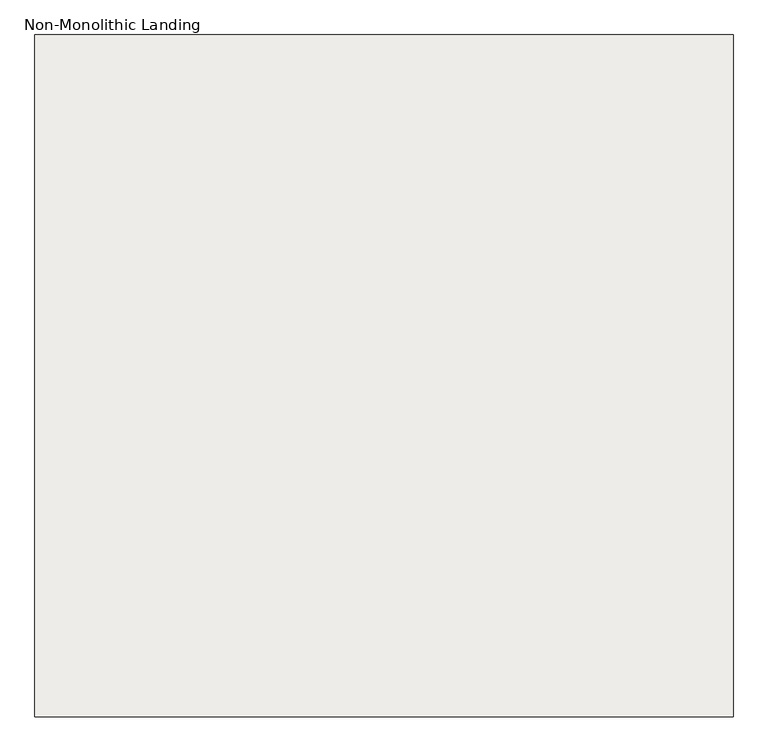
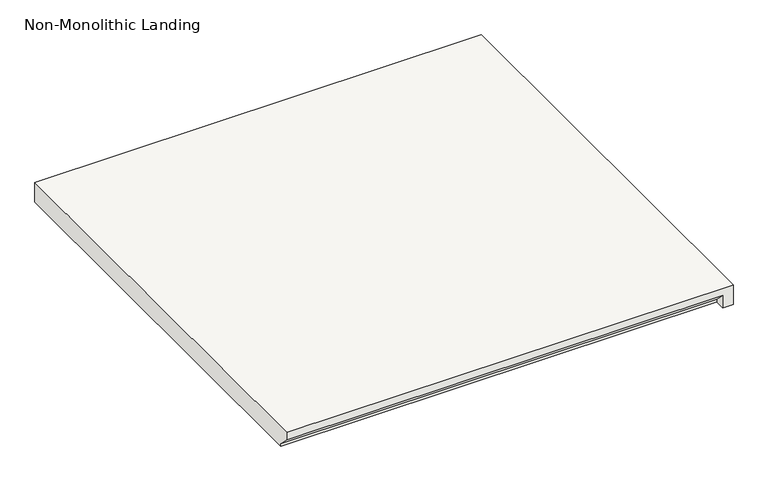
"""IFC4 building model written with IfcOpenShell, lengths in millimetres: slab geometry, Non-Monolithic Landing."""

import ifcopenshell
import ifcopenshell.guid

model = None  # the IFC model being written
_history = None  # IfcOwnerHistory: only IFC2X3 demands one
_inside = {}  # id of a spatial element -> (the spatial element, [elements in it])
_under = {}  # id of a project, library or spatial element -> (it, [spatial elements below it])
_declared = {}  # id of a project -> (the project, [libraries it declares])
_typed = {}  # id of a type object -> (the type object, [elements of that type])
_made_of = {}  # id of a material, layer set ... -> (it, [elements and type objects made of it])


def new_model(schema):
    """Start an empty IFC model of exactly this schema.

    Asked for "IFC4X3", IfcOpenShell would pick the latest addendum, in which some entities
    have other attributes; the version numbers below select the first issue.
    IFC2X3 requires an IfcOwnerHistory on every rooted entity: one is made here for all.
    """
    global model, _history
    if schema == "IFC4X3":
        model = ifcopenshell.file(schema_version=(4, 3, 0, 0))
    else:
        model = ifcopenshell.file(schema=schema)
    _inside.clear()
    _under.clear()
    _declared.clear()
    _typed.clear()
    _made_of.clear()
    _history = None
    if model.schema == "IFC2X3":
        org = make("IfcOrganization", Name="unknown")
        user = make(
            "IfcPersonAndOrganization",
            ThePerson=make("IfcPerson", FamilyName="unknown"),
            TheOrganization=org,
        )
        app = make(
            "IfcApplication",
            ApplicationDeveloper=org,
            Version="unknown",
            ApplicationFullName="unknown",
            ApplicationIdentifier="unknown",
        )
        _history = make(
            "IfcOwnerHistory",
            OwningUser=user,
            OwningApplication=app,
            ChangeAction="ADDED",
            CreationDate=0,
        )
    return model


def make(cls, **values):
    """One entity of the class cls with the attributes given. An attribute that is None is left unset."""
    return model.create_entity(
        cls, **{name: value for name, value in values.items() if value is not None}
    )


def rooted(cls, **values):
    """An entity with a GlobalId (a new one), such as an element, a storey or a relation."""
    return make(cls, GlobalId=ifcopenshell.guid.new(), OwnerHistory=_history, **values)


def si_unit(unit_type, name, prefix=None):
    """IfcSIUnit, for example si_unit("LENGTHUNIT", "METRE", prefix="MILLI")."""
    return make("IfcSIUnit", UnitType=unit_type, Prefix=prefix, Name=name)


def assignment(units):
    """IfcUnitAssignment: the units of a project."""
    return None if units is None else make("IfcUnitAssignment", Units=units)


def point(xyz):
    """IfcCartesianPoint."""
    return None if xyz is None else make("IfcCartesianPoint", Coordinates=xyz)


def direction(xyz):
    """IfcDirection."""
    return None if xyz is None else make("IfcDirection", DirectionRatios=xyz)


def frame(location, z_axis=None, x_axis=None):
    """IfcAxis2Placement3D, a coordinate frame: its origin and axes. An axis left out is left unset."""
    return make(
        "IfcAxis2Placement3D",
        Location=point(location),
        Axis=direction(z_axis),
        RefDirection=direction(x_axis),
    )


def origin():
    """The frame at (0, 0, 0) with its axes left unset."""
    return frame((0.0, 0.0, 0.0))


def place(relative_to, where):
    """IfcLocalPlacement: puts the frame where relative to a parent placement (None: the world)."""
    return make(
        "IfcLocalPlacement", PlacementRelTo=relative_to, RelativePlacement=where
    )


def context(
    kind, dimensions, precision=None, world=None, true_north=None, identifier=None
):
    """IfcGeometricRepresentationContext, for example the 3D "Model" context."""
    return make(
        "IfcGeometricRepresentationContext",
        ContextIdentifier=identifier,
        ContextType=kind,
        CoordinateSpaceDimension=dimensions,
        Precision=precision,
        WorldCoordinateSystem=world,
        TrueNorth=true_north,
    )


def project(units=None, contexts=None):
    """IfcProject with its units and contexts."""
    return rooted(
        "IfcProject",
        Name="project",
        RepresentationContexts=contexts,
        UnitsInContext=assignment(units),
    )


def spatial(cls, under=None, at=None, **own):
    """A site, building, storey or space (cls), placed at a placement, below another one or the project."""
    s = rooted(cls, ObjectPlacement=at, **own)
    if under is not None:
        _under.setdefault(under.id(), (under, []))[1].append(s)
    return s


def faces_of(points, faces, orient=None, outer=None):
    """IfcFace entities. A face is a list of loops; a loop is a list of indices into points, from 0.

    orient and outer hold one flag for each loop. By default every Orientation is true, the
    first loop of a face is its IfcFaceOuterBound and the others are IfcFaceBound.
    """
    made = []
    for i, loops in enumerate(faces):
        bounds = []
        for j, loop in enumerate(loops):
            is_outer = j == 0 if outer is None else outer[i][j]
            bounds.append(
                make(
                    "IfcFaceOuterBound" if is_outer else "IfcFaceBound",
                    Bound=make("IfcPolyLoop", Polygon=[points[k] for k in loop]),
                    Orientation=True if orient is None else orient[i][j],
                )
            )
        made.append(make("IfcFace", Bounds=bounds))
    return made


def faceted_brep(points, faces, orient=None, outer=None, voids=None):
    """IfcFacetedBrep: a solid bounded by flat faces; with voids (closed shells), ...WithVoids."""
    shared = [point(p) for p in points]
    hull = make("IfcClosedShell", CfsFaces=faces_of(shared, faces, orient, outer))
    if voids is None:
        return make("IfcFacetedBrep", Outer=hull)
    return make(
        "IfcFacetedBrepWithVoids",
        Outer=hull,
        Voids=[
            make(cls, CfsFaces=faces_of(shared, fs, o, b)) for cls, fs, o, b in voids
        ],
    )


def shape(context_of_items, identifier, shape_type, items):
    """IfcShapeRepresentation: the items that make up one representation, for example the "Body"."""
    return make(
        "IfcShapeRepresentation",
        ContextOfItems=context_of_items,
        RepresentationIdentifier=identifier,
        RepresentationType=shape_type,
        Items=items,
    )


def source(mapping_origin, context_of_items, identifier, shape_type, items):
    """IfcRepresentationMap: a shape defined once, which mapped items show again and again."""
    return make(
        "IfcRepresentationMap",
        MappingOrigin=mapping_origin,
        MappedRepresentation=shape(context_of_items, identifier, shape_type, items),
    )


def transform(
    local_origin,
    x_axis=None,
    y_axis=None,
    z_axis=None,
    scale=None,
    scale2=None,
    scale3=None,
    uniform=True,
):
    """IfcCartesianTransformationOperator3D, or its non-uniform kind. x_axis, y_axis, z_axis: its Axis1, 2, 3."""
    if uniform:
        return make(
            "IfcCartesianTransformationOperator3D",
            Axis1=direction(x_axis),
            Axis2=direction(y_axis),
            LocalOrigin=point(local_origin),
            Scale=scale,
            Axis3=direction(z_axis),
        )
    return make(
        "IfcCartesianTransformationOperator3DnonUniform",
        Axis1=direction(x_axis),
        Axis2=direction(y_axis),
        LocalOrigin=point(local_origin),
        Scale=scale,
        Axis3=direction(z_axis),
        Scale2=scale2,
        Scale3=scale3,
    )


def mapped(mapping_source, mapping_target):
    """IfcMappedItem: shows the shape of a source again, moved by a transform."""
    return make(
        "IfcMappedItem", MappingSource=mapping_source, MappingTarget=mapping_target
    )


def made_of(thing, what):
    """Note that an element or type object is made of a material, layer set ...; save() writes the relation."""
    if what is not None:
        _made_of.setdefault(what.id(), (what, []))[1].append(thing)
    return thing


def element(
    cls,
    number,
    at=None,
    inside=None,
    cuts=None,
    type_object=None,
    material=None,
    context=None,
    identifier="Body",
    shape_type=None,
    held_by="IfcProductDefinitionShape",
    body=None,
    shapes=None,
    **own,
):
    """One element of the class cls, such as IfcWall. Its Tag is "e" and its number.

    at: its placement. inside: the storey or other place that contains it. cuts: it is an
    opening in that element (IfcRelVoidsElement). A single representation is given by context,
    identifier, shape_type and body (its items); several are given by shapes. held_by: the class
    of the entity that holds the representations. save() writes the other relations.
    """
    e = rooted(cls, Tag="e%d" % number, ObjectPlacement=at, **own)
    if body is not None:
        shapes = [shape(context, identifier, shape_type, body)]
    if shapes is not None:
        e.Representation = make(held_by, Representations=shapes)
    if inside is not None:
        _inside.setdefault(inside.id(), (inside, []))[1].append(e)
    if cuts is not None:
        rooted(
            "IfcRelVoidsElement", RelatingBuildingElement=cuts, RelatedOpeningElement=e
        )
    if type_object is not None:
        _typed.setdefault(type_object.id(), (type_object, []))[1].append(e)
    return made_of(e, material)


def aggregate(whole, parts):
    """IfcRelAggregates: a whole, such as a stair, and the parts it consists of."""
    return rooted("IfcRelAggregates", RelatingObject=whole, RelatedObjects=parts)


def save(model, path):
    """Write the relations noted so far, then the file.

    IfcRelAggregates (storeys below a building ...), IfcRelContainedInSpatialStructure (elements
    in a storey), IfcRelDefinesByType, IfcRelAssociatesMaterial and IfcRelDeclares: one each for
    every whole, place, type object, material and project.
    """
    for whole, parts in _under.values():
        aggregate(whole, parts)
    for where, things in _inside.values():
        rooted(
            "IfcRelContainedInSpatialStructure",
            RelatedElements=things,
            RelatingStructure=where,
        )
    for kind, things in _typed.values():
        rooted("IfcRelDefinesByType", RelatedObjects=things, RelatingType=kind)
    for what, things in _made_of.values():
        rooted("IfcRelAssociatesMaterial", RelatedObjects=things, RelatingMaterial=what)
    for by, libraries in _declared.values():
        rooted("IfcRelDeclares", RelatingContext=by, RelatedDefinitions=libraries)
    model.write(path)


def non_monolithic_landing_abe35be6(model_context):
    return source(origin(), model_context, "Body", "Brep", [
        faceted_brep([(34845.7697162, -5622.8453523, 993.9617647), (34845.7697162, -5597.4453523, 968.5617647), (35912.5697162, -5597.4453523, 968.5617647), (35912.5697162, -5622.8453523, 993.9617647), (35937.9697162, -5622.8453523, 1013.0117647), (35937.9697162, -4556.0453523, 1013.0117647), (35912.5697162, -4556.0453523, 1013.0117647), (34845.7697162, -4556.0453523, 1013.0117647), (34845.7697162, -5622.8453523, 1013.0117647), (35912.5697162, -5597.4453523, 962.2117647), (34845.7697162, -5597.4453523, 962.2117647), (34845.7697162, -4556.0453523, 962.2117647), (35912.5697162, -4556.0453523, 962.2117647), (35937.9697162, -4556.0453523, 962.2117647), (35937.9697162, -5622.8453523, 962.2117647), (35912.5697162, -5622.8453523, 962.2117647)], [[[0, 1, 2, 3]], [[4, 5, 6, 7, 8]], [[9, 10, 11, 12, 13, 14, 15]], [[10, 9, 2, 1]], [[9, 15, 3, 2]], [[4, 8, 0, 3, 15, 14]], [[5, 4, 14, 13]], [[6, 5, 13, 12]], [[7, 6, 12, 11]], [[8, 7, 11, 10, 1, 0]]]),
    ])


if __name__ == "__main__":
    model = new_model("IFC4")
    model_context = context("Model", 3, world=origin())
    ifc_project = project(units=[si_unit("LENGTHUNIT", "METRE", prefix="MILLI")], contexts=[model_context])
    site = spatial("IfcSite", under=ifc_project)
    building = spatial("IfcBuilding", under=site)
    placement = place(None, origin())
    non_monolithic_landing_shape = non_monolithic_landing_abe35be6(model_context)
    element("IfcSlab", 1, ObjectType="Non-Monolithic Landing", at=placement, inside=building, context=model_context, shape_type="MappedRepresentation", body=[
        mapped(non_monolithic_landing_shape, transform((0.0, 0.0, 0.0), x_axis=(1.0, 0.0, 0.0), y_axis=(0.0, 1.0, 0.0), z_axis=(0.0, 0.0, 1.0))),
    ])
    save(model, "model.ifc")

# Revit data of these elements
# Element 1 (IfcSlab, "Non-Monolithic Landing")
#   Materials on its faces: "Oak Flooring"
# Materials
#   "Oak Flooring": class "Wood", colour RGB 216 169 114, transparency 0, Description = "Quercus Rubra", Cost = 0
